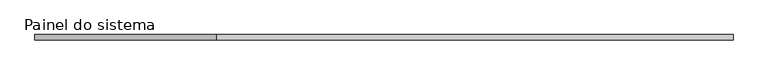
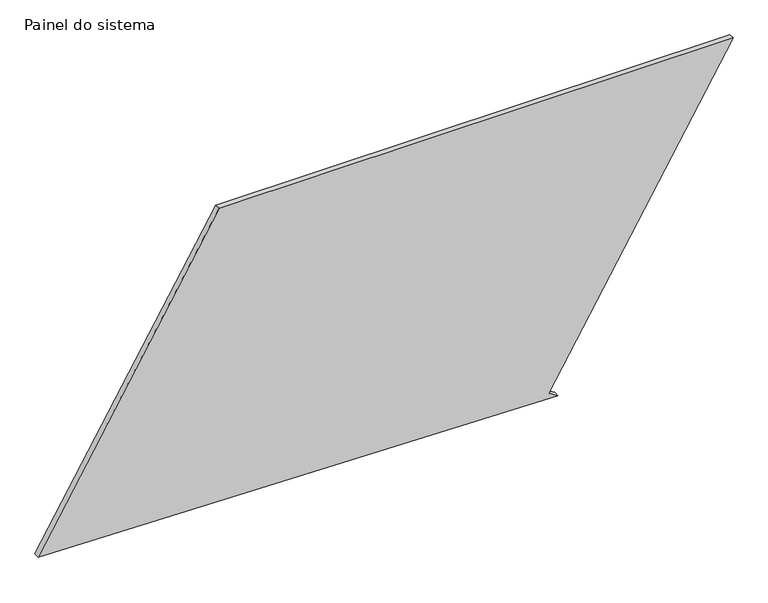
"""IFC4 building model written with IfcOpenShell, lengths in millimetres: plate geometry, Painel do sistema : Envidraçado."""

from ifc_helpers import new_model, si_unit, frame, origin, place, context, project, spatial, polyline, outline, extrude, source, transform, mapped, element, save


def painel_do_sistema_7762b353(model_context):
    return source(origin(), model_context, "Body", "SweptSolid", [
        extrude(outline(polyline([(0.0, 803.3149239), (25.5011879, 760.3069082), (1476.6479709, 1620.7503898), (1476.6479709, -776.3089259), (52.4887553, -1620.7503898), (0.0, 803.3149239)])), frame((0.0, 24.5, 0.0), z_axis=(0.0, 1.0, 0.0), x_axis=(0.0, 0.0, 1.0)), (0.0, 0.0, 1.0), 25.0),
    ])


if __name__ == "__main__":
    model = new_model("IFC4")
    model_context = context("Model", 3, world=origin())
    ifc_project = project(units=[si_unit("LENGTHUNIT", "METRE", prefix="MILLI")], contexts=[model_context])
    site = spatial("IfcSite", under=ifc_project)
    building = spatial("IfcBuilding", under=site)
    placement = place(None, origin())
    painel_do_sistema_shape = painel_do_sistema_7762b353(model_context)
    element("IfcPlate", 1, ObjectType="Painel do sistema : Envidraçado", at=placement, inside=building, context=model_context, shape_type="MappedRepresentation", body=[
        mapped(painel_do_sistema_shape, transform((0.0, 0.0, 0.0), x_axis=(1.0, 0.0, 0.0), y_axis=(0.0, 1.0, 0.0), z_axis=(0.0, 0.0, 1.0))),
    ])
    save(model, "model.ifc")

# Revit data of these elements
# Type "Painel do sistema : Envidraçado"
#   Construction Type Id = "GSP4R"
#   Analytic Construction = "Vidraça única Pilkington 1/8 pol"
#   Visual Light Transmittance = 0.9
#   Solar Heat Gain Coefficient = 0.86
#   Heat Transfer Coefficient (U) = 6.7069 W/(m²·K)
# Element 1 (IfcPlate, "Painel do sistema : Envidraçado")
#   Materials on its faces: "Vidro"
# Materials
#   "Vidro": class "Vidro", colour RGB 0 128 192, transparency 0.9, Description = "Vidro de sílica", Cost = 0
